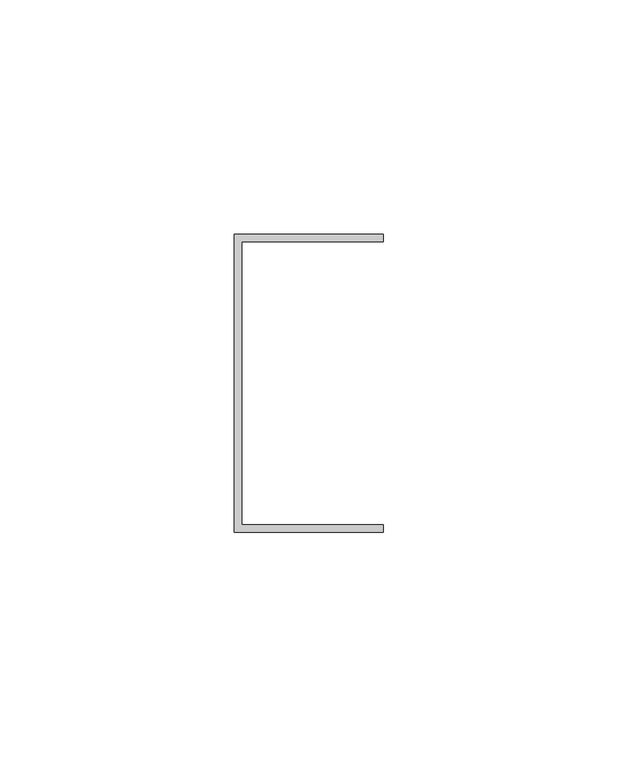
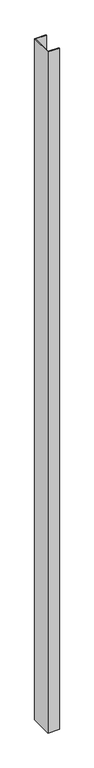
"""IFC4 building model written with IfcOpenShell, lengths in millimetres: proxy geometry, Generic Models 7:Generic Models 1:3:Generic Models 1:3 : Generic Models 7:Generic Models 1:305549:3:Generic Models 1:3:Generic Models 1:3 : Generic Models 7:Generic Models 1:305549:3 : Generic Models 7:Generic Models 1:3:Generic Models 1:3 : Generic Models 7:Generic Models 1:305549:301244:24 : Generic Models 7:Generic Models 1:3:Generic Models 1:3 : Generic Models 7:Generic Models 1:305549:3:Generic Models 1:3:Generic Models 1:3 : Generic Models 7:Generic Models 1:305549:3 : Generic Models 7:Generic Models 1:3:Generic Models 1:3 : Generic Models 7:Generic Models 1:305549:301244:308848."""

import ifcopenshell
import ifcopenshell.guid

model = None  # the IFC model being written
_history = None  # IfcOwnerHistory: only IFC2X3 demands one
_inside = {}  # id of a spatial element -> (the spatial element, [elements in it])
_under = {}  # id of a project, library or spatial element -> (it, [spatial elements below it])
_declared = {}  # id of a project -> (the project, [libraries it declares])
_typed = {}  # id of a type object -> (the type object, [elements of that type])
_made_of = {}  # id of a material, layer set ... -> (it, [elements and type objects made of it])


def new_model(schema):
    """Start an empty IFC model of exactly this schema.

    Asked for "IFC4X3", IfcOpenShell would pick the latest addendum, in which some entities
    have other attributes; the version numbers below select the first issue.
    IFC2X3 requires an IfcOwnerHistory on every rooted entity: one is made here for all.
    """
    global model, _history
    if schema == "IFC4X3":
        model = ifcopenshell.file(schema_version=(4, 3, 0, 0))
    else:
        model = ifcopenshell.file(schema=schema)
    _inside.clear()
    _under.clear()
    _declared.clear()
    _typed.clear()
    _made_of.clear()
    _history = None
    if model.schema == "IFC2X3":
        org = make("IfcOrganization", Name="unknown")
        user = make(
            "IfcPersonAndOrganization",
            ThePerson=make("IfcPerson", FamilyName="unknown"),
            TheOrganization=org,
        )
        app = make(
            "IfcApplication",
            ApplicationDeveloper=org,
            Version="unknown",
            ApplicationFullName="unknown",
            ApplicationIdentifier="unknown",
        )
        _history = make(
            "IfcOwnerHistory",
            OwningUser=user,
            OwningApplication=app,
            ChangeAction="ADDED",
            CreationDate=0,
        )
    return model


def make(cls, **values):
    """One entity of the class cls with the attributes given. An attribute that is None is left unset."""
    return model.create_entity(
        cls, **{name: value for name, value in values.items() if value is not None}
    )


def rooted(cls, **values):
    """An entity with a GlobalId (a new one), such as an element, a storey or a relation."""
    return make(cls, GlobalId=ifcopenshell.guid.new(), OwnerHistory=_history, **values)


def si_unit(unit_type, name, prefix=None):
    """IfcSIUnit, for example si_unit("LENGTHUNIT", "METRE", prefix="MILLI")."""
    return make("IfcSIUnit", UnitType=unit_type, Prefix=prefix, Name=name)


def assignment(units):
    """IfcUnitAssignment: the units of a project."""
    return None if units is None else make("IfcUnitAssignment", Units=units)


def point(xyz):
    """IfcCartesianPoint."""
    return None if xyz is None else make("IfcCartesianPoint", Coordinates=xyz)


def direction(xyz):
    """IfcDirection."""
    return None if xyz is None else make("IfcDirection", DirectionRatios=xyz)


def frame(location, z_axis=None, x_axis=None):
    """IfcAxis2Placement3D, a coordinate frame: its origin and axes. An axis left out is left unset."""
    return make(
        "IfcAxis2Placement3D",
        Location=point(location),
        Axis=direction(z_axis),
        RefDirection=direction(x_axis),
    )


def origin():
    """The frame at (0, 0, 0) with its axes left unset."""
    return frame((0.0, 0.0, 0.0))


def place(relative_to, where):
    """IfcLocalPlacement: puts the frame where relative to a parent placement (None: the world)."""
    return make(
        "IfcLocalPlacement", PlacementRelTo=relative_to, RelativePlacement=where
    )


def context(
    kind, dimensions, precision=None, world=None, true_north=None, identifier=None
):
    """IfcGeometricRepresentationContext, for example the 3D "Model" context."""
    return make(
        "IfcGeometricRepresentationContext",
        ContextIdentifier=identifier,
        ContextType=kind,
        CoordinateSpaceDimension=dimensions,
        Precision=precision,
        WorldCoordinateSystem=world,
        TrueNorth=true_north,
    )


def project(units=None, contexts=None):
    """IfcProject with its units and contexts."""
    return rooted(
        "IfcProject",
        Name="project",
        RepresentationContexts=contexts,
        UnitsInContext=assignment(units),
    )


def spatial(cls, under=None, at=None, **own):
    """A site, building, storey or space (cls), placed at a placement, below another one or the project."""
    s = rooted(cls, ObjectPlacement=at, **own)
    if under is not None:
        _under.setdefault(under.id(), (under, []))[1].append(s)
    return s


def polyline(points):
    """IfcPolyline through the points."""
    return make("IfcPolyline", Points=[point(p) for p in points])


def outline(outer, holes=None, kind="AREA"):
    """IfcArbitraryClosedProfileDef: a profile drawn as a closed curve; with holes, ...WithVoids."""
    if holes is None:
        return make("IfcArbitraryClosedProfileDef", ProfileType=kind, OuterCurve=outer)
    return make(
        "IfcArbitraryProfileDefWithVoids",
        ProfileType=kind,
        OuterCurve=outer,
        InnerCurves=holes,
    )


def extrude(swept, where, along, depth):
    """IfcExtrudedAreaSolid: the profile swept, set in the frame where, extruded along a direction by depth."""
    return make(
        "IfcExtrudedAreaSolid",
        SweptArea=swept,
        Position=where,
        ExtrudedDirection=direction(along),
        Depth=depth,
    )


def shape(context_of_items, identifier, shape_type, items):
    """IfcShapeRepresentation: the items that make up one representation, for example the "Body"."""
    return make(
        "IfcShapeRepresentation",
        ContextOfItems=context_of_items,
        RepresentationIdentifier=identifier,
        RepresentationType=shape_type,
        Items=items,
    )


def source(mapping_origin, context_of_items, identifier, shape_type, items):
    """IfcRepresentationMap: a shape defined once, which mapped items show again and again."""
    return make(
        "IfcRepresentationMap",
        MappingOrigin=mapping_origin,
        MappedRepresentation=shape(context_of_items, identifier, shape_type, items),
    )


def transform(
    local_origin,
    x_axis=None,
    y_axis=None,
    z_axis=None,
    scale=None,
    scale2=None,
    scale3=None,
    uniform=True,
):
    """IfcCartesianTransformationOperator3D, or its non-uniform kind. x_axis, y_axis, z_axis: its Axis1, 2, 3."""
    if uniform:
        return make(
            "IfcCartesianTransformationOperator3D",
            Axis1=direction(x_axis),
            Axis2=direction(y_axis),
            LocalOrigin=point(local_origin),
            Scale=scale,
            Axis3=direction(z_axis),
        )
    return make(
        "IfcCartesianTransformationOperator3DnonUniform",
        Axis1=direction(x_axis),
        Axis2=direction(y_axis),
        LocalOrigin=point(local_origin),
        Scale=scale,
        Axis3=direction(z_axis),
        Scale2=scale2,
        Scale3=scale3,
    )


def mapped(mapping_source, mapping_target):
    """IfcMappedItem: shows the shape of a source again, moved by a transform."""
    return make(
        "IfcMappedItem", MappingSource=mapping_source, MappingTarget=mapping_target
    )


def made_of(thing, what):
    """Note that an element or type object is made of a material, layer set ...; save() writes the relation."""
    if what is not None:
        _made_of.setdefault(what.id(), (what, []))[1].append(thing)
    return thing


def element(
    cls,
    number,
    at=None,
    inside=None,
    cuts=None,
    type_object=None,
    material=None,
    context=None,
    identifier="Body",
    shape_type=None,
    held_by="IfcProductDefinitionShape",
    body=None,
    shapes=None,
    **own,
):
    """One element of the class cls, such as IfcWall. Its Tag is "e" and its number.

    at: its placement. inside: the storey or other place that contains it. cuts: it is an
    opening in that element (IfcRelVoidsElement). A single representation is given by context,
    identifier, shape_type and body (its items); several are given by shapes. held_by: the class
    of the entity that holds the representations. save() writes the other relations.
    """
    e = rooted(cls, Tag="e%d" % number, ObjectPlacement=at, **own)
    if body is not None:
        shapes = [shape(context, identifier, shape_type, body)]
    if shapes is not None:
        e.Representation = make(held_by, Representations=shapes)
    if inside is not None:
        _inside.setdefault(inside.id(), (inside, []))[1].append(e)
    if cuts is not None:
        rooted(
            "IfcRelVoidsElement", RelatingBuildingElement=cuts, RelatedOpeningElement=e
        )
    if type_object is not None:
        _typed.setdefault(type_object.id(), (type_object, []))[1].append(e)
    return made_of(e, material)


def aggregate(whole, parts):
    """IfcRelAggregates: a whole, such as a stair, and the parts it consists of."""
    return rooted("IfcRelAggregates", RelatingObject=whole, RelatedObjects=parts)


def save(model, path):
    """Write the relations noted so far, then the file.

    IfcRelAggregates (storeys below a building ...), IfcRelContainedInSpatialStructure (elements
    in a storey), IfcRelDefinesByType, IfcRelAssociatesMaterial and IfcRelDeclares: one each for
    every whole, place, type object, material and project.
    """
    for whole, parts in _under.values():
        aggregate(whole, parts)
    for where, things in _inside.values():
        rooted(
            "IfcRelContainedInSpatialStructure",
            RelatedElements=things,
            RelatingStructure=where,
        )
    for kind, things in _typed.values():
        rooted("IfcRelDefinesByType", RelatedObjects=things, RelatingType=kind)
    for what, things in _made_of.values():
        rooted("IfcRelAssociatesMaterial", RelatedObjects=things, RelatingMaterial=what)
    for by, libraries in _declared.values():
        rooted("IfcRelDeclares", RelatingContext=by, RelatedDefinitions=libraries)
    model.write(path)


def generic_models_5cf31904(model_context):
    return source(origin(), model_context, "Body", "SweptSolid", [
        extrude(outline(polyline([(560654.5867239, -579013.3913841), (560686.3367239, -579013.3913841), (560686.3367239, -579014.9788841), (560656.1742239, -579014.9788841), (560656.1742239, -579075.3038841), (560686.3367239, -579075.3038841), (560686.3367239, -579076.8913841), (560654.5867239, -579076.8913841), (560654.5867239, -579013.3913841)])), frame((0.0, 0.0, 4133.81326), z_axis=(0.0, 0.0, 1.0), x_axis=(1.0, 0.0, 0.0)), (0.0, 0.0, 1.0), 2000.28674),
    ])


if __name__ == "__main__":
    model = new_model("IFC4")
    model_context = context("Model", 3, world=origin())
    ifc_project = project(units=[si_unit("LENGTHUNIT", "METRE", prefix="MILLI")], contexts=[model_context])
    site = spatial("IfcSite", under=ifc_project)
    building = spatial("IfcBuilding", under=site)
    placement = place(None, origin())
    generic_models_shape = generic_models_5cf31904(model_context)
    element("IfcBuildingElementProxy", 1, Name="Generic Models 7:Generic Models 1:3:Generic Models 1:3 : Generic Models 7:Generic Models 1:305549:3:Generic Models 1:3:Generic Models 1:3 : Generic Models 7:Generic Models 1:305549:3 : Generic Models 7:Generic Models 1:3:Generic Models 1:3 : Generic Models 7:Generic Models 1:305549:301244:24 : Generic Models 7:Generic Models 1:3:Generic Models 1:3 : Generic Models 7:Generic Models 1:305549:3:Generic Models 1:3:Generic Models 1:3 : Generic Models 7:Generic Models 1:305549:3 : Generic Models 7:Generic Models 1:3:Generic Models 1:3 : Generic Models 7:Generic Models 1:305549:301244:308848", ObjectType="Generic Models 7:Generic Models 1:3:Generic Models 1:3 : Generic Models 7:Generic Models 1:305549:3:Generic Models 1:3:Generic Models 1:3 : Generic Models 7:Generic Models 1:305549:3 : Generic Models 7:Generic Models 1:3:Generic Models 1:3 : Generic Models 7:Generic Models 1:305549:301244:24 : Generic Models 7:Generic Models 1:3:Generic Models 1:3 : Generic Models 7:Generic Models 1:305549:3:Generic Models 1:3:Generic Models 1:3 : Generic Models 7:Generic Models 1:305549:3 : Generic Models 7:Generic Models 1:3:Generic Models 1:3 : Generic Models 7:Generic Models 1:305549:301244:308848", at=placement, inside=building, context=model_context, shape_type="MappedRepresentation", body=[
        mapped(generic_models_shape, transform((0.0, 0.0, 0.0), x_axis=(1.0, 0.0, 0.0), y_axis=(0.0, 1.0, 0.0), z_axis=(0.0, 0.0, 1.0))),
    ])
    save(model, "model.ifc")

# Revit data of these elements
# Type "Generic Models 7:Generic Models 1:3:Generic Models 1:3 : Generic Models 7:Generic Models 1:305549:3:Generic Models 1:3:Generic Models 1:3 : Generic Models 7:Generic Models 1:305549:3 : Generic Models 7:Generic Models 1:3:Generic Models 1:3 : Generic Models 7:Generic Models 1:305549:301244:24 : Generic Models 7:Generic Models 1:3:Generic Models 1:3 : Generic Models 7:Generic Models 1:305549:3:Generic Models 1:3:Generic Models 1:3 : Generic Models 7:Generic Models 1:305549:3 : Generic Models 7:Generic Models 1:3:Generic Models 1:3 : Generic Models 7:Generic Models 1:305549:301244:308848"
#   NameOverride = "Generic Models 7:Generic Models 1:3:Generic Models 1:3 : Generic Models 7:Generic Models 1:305549:3:Generic Models 1:3:Generic Models 1:3 : Generic Models 7:Generic Models 1:305549:3 : Generic Models 7:Generic Models 1:3:Generic Models 1:3 : Generic Models 7:Generic Models 1:305549:301244:308848"
#   ObjectTypeOverride = "Generic Models 1:3:Generic Models 1:3 : Generic Models 7:Generic Models 1:305549:3 : Generic Models 7:Generic Models 1:3:Generic Models 1:3 : Generic Models 7:Generic Models 1:305549:301244"
#   Reference = "Generic Models 1"
#   Tag = "308848"
# Element 1 (IfcBuildingElementProxy, "Generic Models 7:Generic Models 1:3:Generic Models 1:3 : Generic Models 7:Generic Models 1:305549:3:Generic Models 1:3:Generic Models 1:3 : Generic Models 7:Generic Models 1:305549:3 : Generic Models 7:Generic Models 1:3:Generic Models 1:3 : Generic Models 7:Generic Models 1:305549:301244:24 : Generic Models 7:Generic Models 1:3:Generic Models 1:3 : Generic Models 7:Generic Models 1:305549:3:Generic Models 1:3:Generic Models 1:3 : Generic Models 7:Generic Models 1:305549:3 : Generic Models 7:Generic Models 1:3:Generic Models 1:3 : Generic Models 7:Generic Models 1:305549:301244:308848")
#   Materials on its faces: "GALVANIZED U-CHANNEL (250T125-33)"
# Materials
#   "GALVANIZED U-CHANNEL (250T125-33)": class "Unassigned", colour RGB 202 201 200, transparency 0, Keynote = "M05451300.02", Cost = 0
